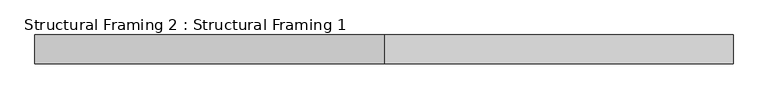
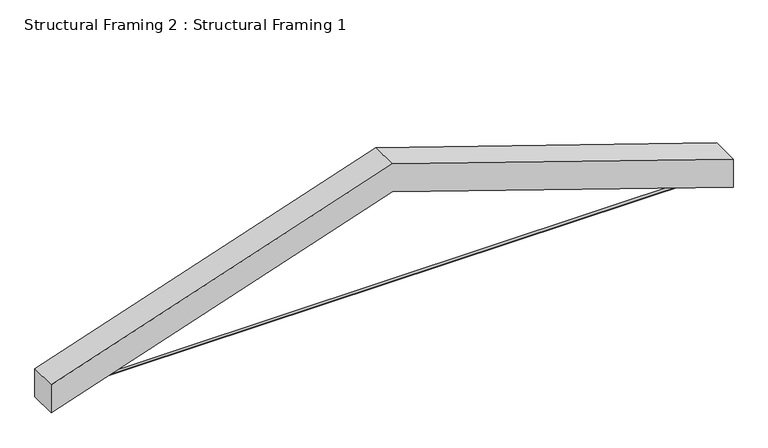
"""IFC4 building model written with IfcOpenShell, lengths in millimetres: beam geometry, Structural Framing 2 : Structural Framing 1."""

from ifc_helpers import new_model, si_unit, point, frame, frame_2d, origin, place, context, project, spatial, polyline, circle_curve, trimmed, segment, composite_curve, outline, extrude, source, transform, mapped, element, save


def structural_framing_2_structural_framing_1_d36d69be(model_context):
    return source(origin(), model_context, "Body", "SweptSolid", [
        extrude(outline(composite_curve([segment(trimmed(circle_curve(frame_2d((1391.9115366, 4984.3019529)), 6.35), [point((1398.2615366, 4984.3019529))], [point((1385.5615366, 4984.3019529))], False, "CARTESIAN"), True, "CONTINUOUS"), segment(trimmed(circle_curve(frame_2d((1391.9115366, 4984.3019529)), 6.35), [point((1385.5615366, 4984.3019529))], [point((1398.2615366, 4984.3019529))], False, "CARTESIAN"), True, "CONTINUOUS")], self_intersect=False)), frame((19888.9870052, 0.0, 0.0), z_axis=(1.0, 0.0, 0.0), x_axis=(0.0, 1.0, 0.0)), (0.0, 0.0, 1.0), 3111.5),
        extrude(outline(polyline([(5652.475838, 21444.7370052), (5084.8528105, 19749.2870052), (4937.5315162, 19749.2870052), (5505.1545437, 21444.7370052), (4937.5315162, 23140.1870052), (5084.8528105, 23140.1870052), (5652.475838, 21444.7370052)])), frame((0.0, 1322.0615366, 0.0), z_axis=(0.0, 1.0, 0.0), x_axis=(0.0, 0.0, 1.0)), (0.0, 0.0, 1.0), 139.7),
    ])


if __name__ == "__main__":
    model = new_model("IFC4")
    model_context = context("Model", 3, world=origin())
    ifc_project = project(units=[si_unit("LENGTHUNIT", "METRE", prefix="MILLI")], contexts=[model_context])
    site = spatial("IfcSite", under=ifc_project)
    building = spatial("IfcBuilding", under=site)
    placement = place(None, origin())
    structural_framing_2_structural_framing_1_shape = structural_framing_2_structural_framing_1_d36d69be(model_context)
    element("IfcBeam", 1, ObjectType="Structural Framing 2 : Structural Framing 1", at=placement, inside=building, context=model_context, shape_type="MappedRepresentation", body=[
        mapped(structural_framing_2_structural_framing_1_shape, transform((0.0, 0.0, 0.0), x_axis=(1.0, 0.0, 0.0), y_axis=(0.0, 1.0, 0.0), z_axis=(0.0, 0.0, 1.0))),
    ])
    save(model, "model.ifc")

# Revit data of these elements
# Element 1 (IfcBeam, "Structural Framing 2 : Structural Framing 1")
#   Materials on its faces: "GLULAM TRUSS W/ CUSTOM GUSSET PLATES", "COLLAR TIE: 1/2\" GALV. ROD"
# Materials
#   "GLULAM TRUSS W/ CUSTOM GUSSET PLATES": class "Generic", colour RGB 206 153 90, transparency 0, Cost = 0
#   "COLLAR TIE: 1/2\" GALV. ROD": class "Generic", colour RGB 49 49 49, transparency 0, Cost = 0
